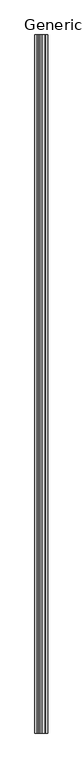
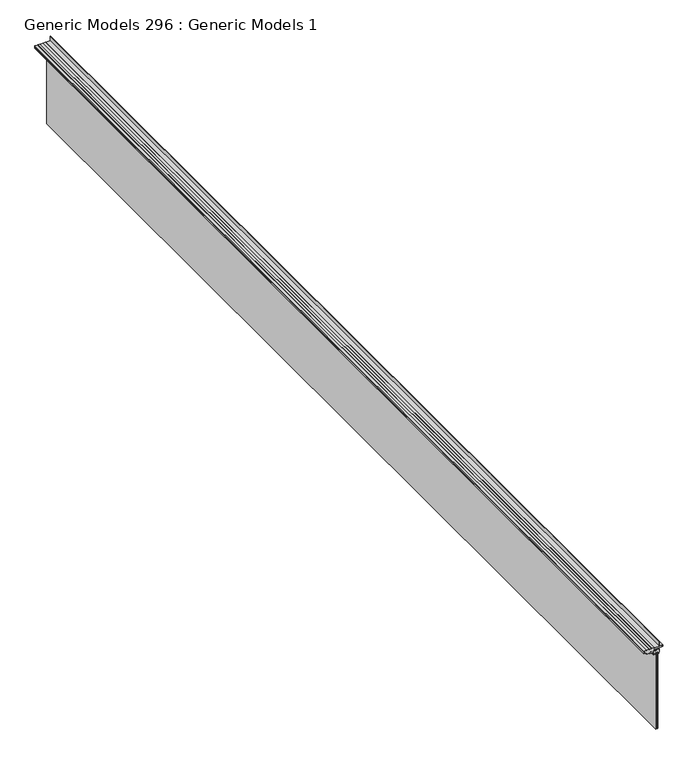
"""IFC4 building model written with IfcOpenShell, lengths in millimetres: proxy geometry, Generic Models 296 : Generic Models 1."""

from ifc_helpers import new_model, si_unit, point, frame, frame_2d, origin, place, context, project, spatial, polyline, circle_curve, trimmed, segment, composite_curve, outline, extrude, source, transform, mapped, element, save


def generic_models_296_generic_models_1_245af7ca(model_context):
    return source(origin(), model_context, "Body", "SweptSolid", [
        extrude(outline(composite_curve([segment(polyline([(124404.9673941, 3535.0400913), (124397.0171769, 3535.0400913), (124397.0171769, 3542.9902843), (124395.0359993, 3542.9902843), (124395.0359993, 3535.0400913), (124385.1045803, 3535.0400913), (124385.1045803, 3545.3524463), (124384.2917908, 3546.1398982), (124384.2917908, 3549.3148982), (124380.3293873, 3549.3148982), (124380.3293873, 3550.9150913), (124377.1543873, 3554.8520603), (124377.1543873, 3556.4522533), (124374.7667908, 3556.4522533), (124374.7667908, 3575.5022533), (124368.4349583, 3575.5022533), (124368.4349583, 3604.9154773), (124371.6099583, 3604.9154773), (124371.6099583, 3601.8675044), (124380.2967583, 3601.8675044), (124380.2967583, 3584.3415044), (124382.5827583, 3584.3415044), (124382.5827583, 3601.8675044), (124383.5225548, 3601.8675044), (124383.5225548, 3610.2748401), (124391.4727478, 3610.2748401), (124391.4727478, 3612.2561145), (124385.0538083, 3612.2561145), (124385.0538083, 3616.2692417), (124389.9306009, 3616.2692417), (124389.9306009, 3651.2196417), (124392.3529708, 3679.0834417), (124401.2843941, 3679.0834417), (124401.2843941, 3671.1798761), (124403.5703941, 3671.1798761), (124403.5703941, 3677.5298761), (124404.9673941, 3677.5298761), (124404.9673941, 3652.6420417), (124440.3344811, 3652.6420417)]), True, "CONTINUOUS"), segment(trimmed(circle_curve(frame_2d((124440.3369408, 3651.9435419)), 0.6985041), [point((124440.3344811, 3652.6420417))], [point((124440.3392817, 3651.2450417))], False, "CARTESIAN"), True, "CONTINUOUS"), segment(polyline([(124440.3392817, 3651.2450417), (124404.9673941, 3651.2450417), (124404.9673941, 3614.7758738), (124401.7923941, 3614.7758738), (124401.7923941, 3612.4898738), (124404.9673941, 3612.4898738), (124404.9673941, 3595.3904913), (124402.8845941, 3595.3904913), (124402.8845941, 3592.2154913), (124404.9673941, 3592.2154913), (124404.9673941, 3575.1883916), (124401.7923941, 3575.1883916), (124401.7923941, 3572.9023877), (124404.9673941, 3572.9023877), (124404.9673941, 3555.3946386), (124401.7923941, 3555.3946386), (124401.7923941, 3553.1086347), (124404.9673941, 3553.1086347), (124404.9673941, 3535.0400913)]), True, "CONTINUOUS")], self_intersect=False)), frame((0.0, -1504.2676118, 0.0), z_axis=(0.0, 1.0, 0.0), x_axis=(0.0, 0.0, 1.0)), (0.0, 0.0, 1.0), 7886.7),
        extrude(outline(composite_curve([segment(polyline([(124356.1104833, 3642.7431837), (124351.8750441, 3642.7431837), (124351.8750441, 3643.8790417), (124349.8486703, 3643.8790417), (124350.0382206, 3646.3220811), (124357.8440441, 3648.8574417), (124357.8440441, 3651.2450417), (124380.1452441, 3651.2450417)]), True, "CONTINUOUS"), segment(trimmed(circle_curve(frame_2d((124380.1452441, 3648.8574417)), 2.3876), [point((124380.1452441, 3651.2450417))], [point((124382.5328441, 3648.8574417))], False, "CARTESIAN"), True, "CONTINUOUS"), segment(polyline([(124382.5328441, 3648.8574417), (124382.5328441, 3646.2920417), (124380.5008441, 3646.2920417), (124380.5008441, 3644.6156417), (124377.1988441, 3644.6156417), (124377.1988441, 3642.7106417), (124385.1236441, 3642.7106417), (124385.1236441, 3637.0972417), (124379.8150441, 3637.0972417), (124379.8150441, 3624.9052417)]), True, "CONTINUOUS"), segment(trimmed(circle_curve(frame_2d((124379.8150441, 3622.9240417)), 1.9812), [point((124379.8150441, 3624.9052417))], [point((124379.8150441, 3620.9428417))], True, "CARTESIAN"), True, "CONTINUOUS"), segment(polyline([(124379.8150441, 3620.9428417), (124379.8150441, 3607.6078417)]), True, "CONTINUOUS"), segment(trimmed(circle_curve(frame_2d((124379.0022441, 3607.6078417)), 0.8128), [point((124379.8150441, 3607.6078417))], [point((124379.0022441, 3606.7950417))], False, "CARTESIAN"), True, "CONTINUOUS"), segment(polyline([(124379.0022441, 3606.7950417), (124360.7142441, 3606.7950417), (124360.7142441, 3608.6755596), (124359.1133553, 3608.6755596), (124359.1133553, 3607.0753596), (124351.5695553, 3607.0753596), (124351.5695553, 3610.8432792), (124349.4072053, 3610.8432792), (124348.3945553, 3622.6709596), (124358.3259553, 3622.6709596), (124360.7142441, 3620.2826708), (124360.7142441, 3641.7200417), (124357.1336253, 3641.7200417), (124356.1104833, 3642.7431837)]), True, "CONTINUOUS")], self_intersect=False)), frame((0.0, -1504.2676118, 0.0), z_axis=(0.0, 1.0, 0.0), x_axis=(0.0, 0.0, 1.0)), (0.0, 0.0, 1.0), 7886.7),
        extrude(outline(polyline([(3628.2272096, -1504.2676118), (3623.4647096, -1504.2676118), (3623.4647096, 6382.4323882), (3628.2272096, 6382.4323882), (3628.2272096, -1504.2676118)])), frame((0.0, 0.0, 123757.582946), z_axis=(0.0, 0.0, 1.0), x_axis=(1.0, 0.0, 0.0)), (0.0, 0.0, 1.0), 602.3375481),
        extrude(outline(polyline([(3635.3700417, -1504.2676118), (3629.0209596, -1504.2676118), (3629.0209596, 6382.4323882), (3635.3700417, 6382.4323882), (3635.3700417, -1504.2676118)])), frame((0.0, 0.0, 124353.5704941), z_axis=(0.0, 0.0, 1.0), x_axis=(1.0, 0.0, 0.0)), (0.0, 0.0, 1.0), 6.35),
        extrude(outline(polyline([(3640.9262917, -1504.2676118), (3636.1637917, -1504.2676118), (3636.1637917, 6382.4323882), (3640.9262917, 6382.4323882), (3640.9262917, -1504.2676118)])), frame((0.0, 0.0, 123757.582946), z_axis=(0.0, 0.0, 1.0), x_axis=(1.0, 0.0, 0.0)), (0.0, 0.0, 1.0), 602.3375481),
    ])


if __name__ == "__main__":
    model = new_model("IFC4")
    model_context = context("Model", 3, world=origin())
    ifc_project = project(units=[si_unit("LENGTHUNIT", "METRE", prefix="MILLI")], contexts=[model_context])
    site = spatial("IfcSite", under=ifc_project)
    building = spatial("IfcBuilding", under=site)
    placement = place(None, origin())
    generic_models_296_generic_models_1_shape = generic_models_296_generic_models_1_245af7ca(model_context)
    element("IfcBuildingElementProxy", 1, Name="Generic Models 296 : Generic Models 1", ObjectType="Generic Models 296 : Generic Models 1", at=placement, inside=building, context=model_context, shape_type="MappedRepresentation", body=[
        mapped(generic_models_296_generic_models_1_shape, transform((0.0, 0.0, 0.0), x_axis=(1.0, 0.0, 0.0), y_axis=(0.0, 1.0, 0.0), z_axis=(0.0, 0.0, 1.0))),
    ])
    save(model, "model.ifc")

# Revit data of these elements
# Element 1 (IfcBuildingElementProxy, "Generic Models 296 : Generic Models 1")
#   Materials on its faces: "_WINDOW PER SCHEDULE"
# Materials
#   "_WINDOW PER SCHEDULE": class "Generic", colour RGB 255 255 255, transparency 0, Cost = 0
